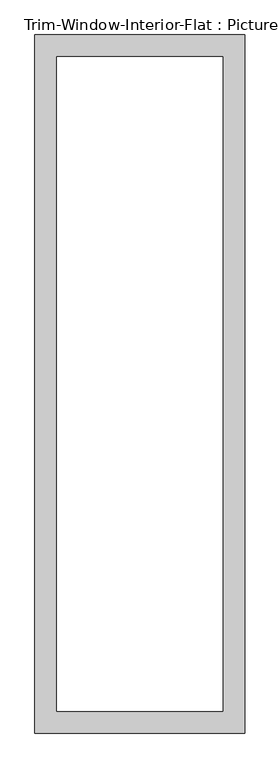
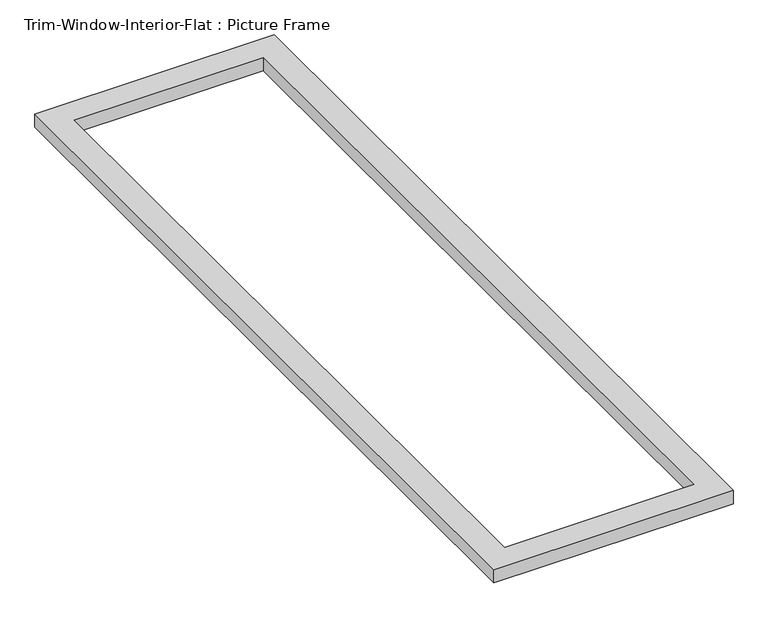
"""IFC4 building model written with IfcOpenShell, lengths in millimetres: proxy geometry, Trim-Window-Interior-Flat : Picture Frame."""

import ifcopenshell
import ifcopenshell.guid

model = None  # the IFC model being written
_history = None  # IfcOwnerHistory: only IFC2X3 demands one
_inside = {}  # id of a spatial element -> (the spatial element, [elements in it])
_under = {}  # id of a project, library or spatial element -> (it, [spatial elements below it])
_declared = {}  # id of a project -> (the project, [libraries it declares])
_typed = {}  # id of a type object -> (the type object, [elements of that type])
_made_of = {}  # id of a material, layer set ... -> (it, [elements and type objects made of it])


def new_model(schema):
    """Start an empty IFC model of exactly this schema.

    Asked for "IFC4X3", IfcOpenShell would pick the latest addendum, in which some entities
    have other attributes; the version numbers below select the first issue.
    IFC2X3 requires an IfcOwnerHistory on every rooted entity: one is made here for all.
    """
    global model, _history
    if schema == "IFC4X3":
        model = ifcopenshell.file(schema_version=(4, 3, 0, 0))
    else:
        model = ifcopenshell.file(schema=schema)
    _inside.clear()
    _under.clear()
    _declared.clear()
    _typed.clear()
    _made_of.clear()
    _history = None
    if model.schema == "IFC2X3":
        org = make("IfcOrganization", Name="unknown")
        user = make(
            "IfcPersonAndOrganization",
            ThePerson=make("IfcPerson", FamilyName="unknown"),
            TheOrganization=org,
        )
        app = make(
            "IfcApplication",
            ApplicationDeveloper=org,
            Version="unknown",
            ApplicationFullName="unknown",
            ApplicationIdentifier="unknown",
        )
        _history = make(
            "IfcOwnerHistory",
            OwningUser=user,
            OwningApplication=app,
            ChangeAction="ADDED",
            CreationDate=0,
        )
    return model


def make(cls, **values):
    """One entity of the class cls with the attributes given. An attribute that is None is left unset."""
    return model.create_entity(
        cls, **{name: value for name, value in values.items() if value is not None}
    )


def rooted(cls, **values):
    """An entity with a GlobalId (a new one), such as an element, a storey or a relation."""
    return make(cls, GlobalId=ifcopenshell.guid.new(), OwnerHistory=_history, **values)


def si_unit(unit_type, name, prefix=None):
    """IfcSIUnit, for example si_unit("LENGTHUNIT", "METRE", prefix="MILLI")."""
    return make("IfcSIUnit", UnitType=unit_type, Prefix=prefix, Name=name)


def assignment(units):
    """IfcUnitAssignment: the units of a project."""
    return None if units is None else make("IfcUnitAssignment", Units=units)


def point(xyz):
    """IfcCartesianPoint."""
    return None if xyz is None else make("IfcCartesianPoint", Coordinates=xyz)


def direction(xyz):
    """IfcDirection."""
    return None if xyz is None else make("IfcDirection", DirectionRatios=xyz)


def frame(location, z_axis=None, x_axis=None):
    """IfcAxis2Placement3D, a coordinate frame: its origin and axes. An axis left out is left unset."""
    return make(
        "IfcAxis2Placement3D",
        Location=point(location),
        Axis=direction(z_axis),
        RefDirection=direction(x_axis),
    )


def origin():
    """The frame at (0, 0, 0) with its axes left unset."""
    return frame((0.0, 0.0, 0.0))


def origin_with_axes():
    """The frame at (0, 0, 0) with the z axis (0, 0, 1) and the x axis (1, 0, 0) written out."""
    return frame((0.0, 0.0, 0.0), z_axis=(0.0, 0.0, 1.0), x_axis=(1.0, 0.0, 0.0))


def place(relative_to, where):
    """IfcLocalPlacement: puts the frame where relative to a parent placement (None: the world)."""
    return make(
        "IfcLocalPlacement", PlacementRelTo=relative_to, RelativePlacement=where
    )


def context(
    kind, dimensions, precision=None, world=None, true_north=None, identifier=None
):
    """IfcGeometricRepresentationContext, for example the 3D "Model" context."""
    return make(
        "IfcGeometricRepresentationContext",
        ContextIdentifier=identifier,
        ContextType=kind,
        CoordinateSpaceDimension=dimensions,
        Precision=precision,
        WorldCoordinateSystem=world,
        TrueNorth=true_north,
    )


def project(units=None, contexts=None):
    """IfcProject with its units and contexts."""
    return rooted(
        "IfcProject",
        Name="project",
        RepresentationContexts=contexts,
        UnitsInContext=assignment(units),
    )


def spatial(cls, under=None, at=None, **own):
    """A site, building, storey or space (cls), placed at a placement, below another one or the project."""
    s = rooted(cls, ObjectPlacement=at, **own)
    if under is not None:
        _under.setdefault(under.id(), (under, []))[1].append(s)
    return s


def polyline(points):
    """IfcPolyline through the points."""
    return make("IfcPolyline", Points=[point(p) for p in points])


def outline(outer, holes=None, kind="AREA"):
    """IfcArbitraryClosedProfileDef: a profile drawn as a closed curve; with holes, ...WithVoids."""
    if holes is None:
        return make("IfcArbitraryClosedProfileDef", ProfileType=kind, OuterCurve=outer)
    return make(
        "IfcArbitraryProfileDefWithVoids",
        ProfileType=kind,
        OuterCurve=outer,
        InnerCurves=holes,
    )


def extrude(swept, where, along, depth):
    """IfcExtrudedAreaSolid: the profile swept, set in the frame where, extruded along a direction by depth."""
    return make(
        "IfcExtrudedAreaSolid",
        SweptArea=swept,
        Position=where,
        ExtrudedDirection=direction(along),
        Depth=depth,
    )


def shape(context_of_items, identifier, shape_type, items):
    """IfcShapeRepresentation: the items that make up one representation, for example the "Body"."""
    return make(
        "IfcShapeRepresentation",
        ContextOfItems=context_of_items,
        RepresentationIdentifier=identifier,
        RepresentationType=shape_type,
        Items=items,
    )


def source(mapping_origin, context_of_items, identifier, shape_type, items):
    """IfcRepresentationMap: a shape defined once, which mapped items show again and again."""
    return make(
        "IfcRepresentationMap",
        MappingOrigin=mapping_origin,
        MappedRepresentation=shape(context_of_items, identifier, shape_type, items),
    )


def transform(
    local_origin,
    x_axis=None,
    y_axis=None,
    z_axis=None,
    scale=None,
    scale2=None,
    scale3=None,
    uniform=True,
):
    """IfcCartesianTransformationOperator3D, or its non-uniform kind. x_axis, y_axis, z_axis: its Axis1, 2, 3."""
    if uniform:
        return make(
            "IfcCartesianTransformationOperator3D",
            Axis1=direction(x_axis),
            Axis2=direction(y_axis),
            LocalOrigin=point(local_origin),
            Scale=scale,
            Axis3=direction(z_axis),
        )
    return make(
        "IfcCartesianTransformationOperator3DnonUniform",
        Axis1=direction(x_axis),
        Axis2=direction(y_axis),
        LocalOrigin=point(local_origin),
        Scale=scale,
        Axis3=direction(z_axis),
        Scale2=scale2,
        Scale3=scale3,
    )


def mapped(mapping_source, mapping_target):
    """IfcMappedItem: shows the shape of a source again, moved by a transform."""
    return make(
        "IfcMappedItem", MappingSource=mapping_source, MappingTarget=mapping_target
    )


def made_of(thing, what):
    """Note that an element or type object is made of a material, layer set ...; save() writes the relation."""
    if what is not None:
        _made_of.setdefault(what.id(), (what, []))[1].append(thing)
    return thing


def element(
    cls,
    number,
    at=None,
    inside=None,
    cuts=None,
    type_object=None,
    material=None,
    context=None,
    identifier="Body",
    shape_type=None,
    held_by="IfcProductDefinitionShape",
    body=None,
    shapes=None,
    **own,
):
    """One element of the class cls, such as IfcWall. Its Tag is "e" and its number.

    at: its placement. inside: the storey or other place that contains it. cuts: it is an
    opening in that element (IfcRelVoidsElement). A single representation is given by context,
    identifier, shape_type and body (its items); several are given by shapes. held_by: the class
    of the entity that holds the representations. save() writes the other relations.
    """
    e = rooted(cls, Tag="e%d" % number, ObjectPlacement=at, **own)
    if body is not None:
        shapes = [shape(context, identifier, shape_type, body)]
    if shapes is not None:
        e.Representation = make(held_by, Representations=shapes)
    if inside is not None:
        _inside.setdefault(inside.id(), (inside, []))[1].append(e)
    if cuts is not None:
        rooted(
            "IfcRelVoidsElement", RelatingBuildingElement=cuts, RelatedOpeningElement=e
        )
    if type_object is not None:
        _typed.setdefault(type_object.id(), (type_object, []))[1].append(e)
    return made_of(e, material)


def aggregate(whole, parts):
    """IfcRelAggregates: a whole, such as a stair, and the parts it consists of."""
    return rooted("IfcRelAggregates", RelatingObject=whole, RelatedObjects=parts)


def save(model, path):
    """Write the relations noted so far, then the file.

    IfcRelAggregates (storeys below a building ...), IfcRelContainedInSpatialStructure (elements
    in a storey), IfcRelDefinesByType, IfcRelAssociatesMaterial and IfcRelDeclares: one each for
    every whole, place, type object, material and project.
    """
    for whole, parts in _under.values():
        aggregate(whole, parts)
    for where, things in _inside.values():
        rooted(
            "IfcRelContainedInSpatialStructure",
            RelatedElements=things,
            RelatingStructure=where,
        )
    for kind, things in _typed.values():
        rooted("IfcRelDefinesByType", RelatedObjects=things, RelatingType=kind)
    for what, things in _made_of.values():
        rooted("IfcRelAssociatesMaterial", RelatedObjects=things, RelatingMaterial=what)
    for by, libraries in _declared.values():
        rooted("IfcRelDeclares", RelatingContext=by, RelatedDefinitions=libraries)
    model.write(path)


def trim_window_interior_flat_picture_frame_db28ea87(model_context):
    return source(origin(), model_context, "Body", "SweptSolid", [
        extrude(outline(polyline([(273.05, 44.45), (273.05, -1771.65), (-273.05, -1771.65), (-273.05, 44.45), (273.05, 44.45)]), holes=[polyline([(215.9, -12.7), (-215.9, -12.7), (-215.9, -1714.5), (215.9, -1714.5), (215.9, -12.7)])]), origin_with_axes(), (0.0, 0.0, 1.0), 31.75),
    ])


if __name__ == "__main__":
    model = new_model("IFC4")
    model_context = context("Model", 3, world=origin())
    ifc_project = project(units=[si_unit("LENGTHUNIT", "METRE", prefix="MILLI")], contexts=[model_context])
    site = spatial("IfcSite", under=ifc_project)
    building = spatial("IfcBuilding", under=site)
    placement = place(None, origin())
    trim_window_interior_flat_picture_frame_shape = trim_window_interior_flat_picture_frame_db28ea87(model_context)
    element("IfcBuildingElementProxy", 1, Name="Trim-Window-Interior-Flat : Picture Frame", ObjectType="Trim-Window-Interior-Flat : Picture Frame", at=placement, inside=building, context=model_context, shape_type="MappedRepresentation", body=[
        mapped(trim_window_interior_flat_picture_frame_shape, transform((0.0, 0.0, 0.0), x_axis=(1.0, 0.0, 0.0), y_axis=(0.0, 1.0, 0.0), z_axis=(0.0, 0.0, 1.0))),
    ])
    save(model, "model.ifc")

# Revit data of these elements
# Type "Trim-Window-Interior-Flat : Picture Frame"
#   Trim Thickness_Picture Frame = 0' - 1 1/4"
#   Trim Width = 0' - 2 1/4"
#   Trim Thickness_with Sill = 0' - 0 3/4"
#   Sill Thickness = 0' - 1 1/4"
#   Opening Width [instance default] = 2' - 0"
#   Opening Height [instance default] = 3' - 0"
#   Default Elevation = 4' - 0"
#   Sill = no
#   Picture Frame = yes
#   Trim Material [instance default] = none
# Element 1 (IfcBuildingElementProxy, "Trim-Window-Interior-Flat : Picture Frame")
#   Opening Width = 1' - 6"
#   Opening Height = 5' - 8"
#   Trim Material = 1X WOOD COMPOSITE TRIM
#   Materials on its faces: "1X WOOD COMPOSITE TRIM"
# Materials
#   "1X WOOD COMPOSITE TRIM": class "Generic", colour RGB 88 61 61, transparency 0, Cost = 0
